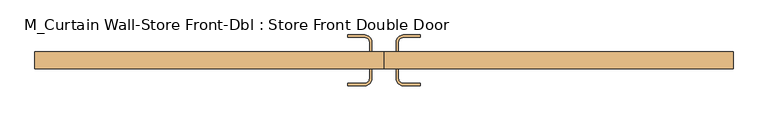
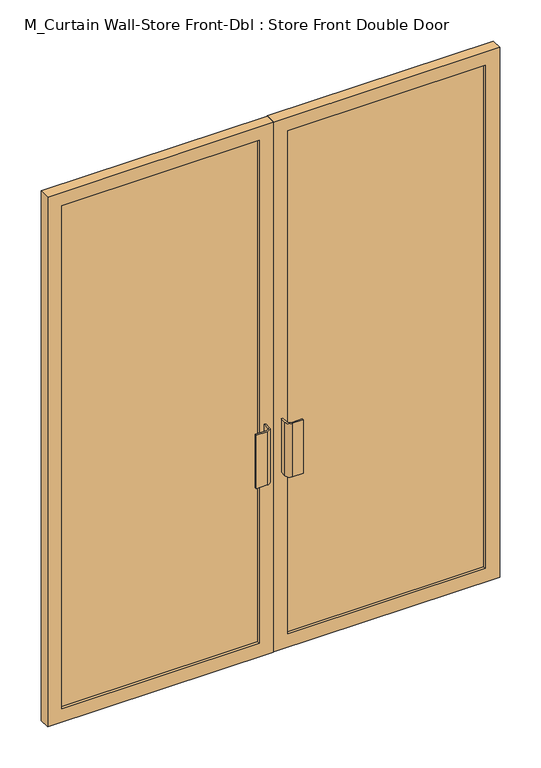
"""IFC4 building model written with IfcOpenShell, lengths in millimetres: door geometry, M_Curtain Wall-Store Front-Dbl : Store Front Double Door."""

import ifcopenshell
import ifcopenshell.guid

model = None  # the IFC model being written
_history = None  # IfcOwnerHistory: only IFC2X3 demands one
_inside = {}  # id of a spatial element -> (the spatial element, [elements in it])
_under = {}  # id of a project, library or spatial element -> (it, [spatial elements below it])
_declared = {}  # id of a project -> (the project, [libraries it declares])
_typed = {}  # id of a type object -> (the type object, [elements of that type])
_made_of = {}  # id of a material, layer set ... -> (it, [elements and type objects made of it])


def new_model(schema):
    """Start an empty IFC model of exactly this schema.

    Asked for "IFC4X3", IfcOpenShell would pick the latest addendum, in which some entities
    have other attributes; the version numbers below select the first issue.
    IFC2X3 requires an IfcOwnerHistory on every rooted entity: one is made here for all.
    """
    global model, _history
    if schema == "IFC4X3":
        model = ifcopenshell.file(schema_version=(4, 3, 0, 0))
    else:
        model = ifcopenshell.file(schema=schema)
    _inside.clear()
    _under.clear()
    _declared.clear()
    _typed.clear()
    _made_of.clear()
    _history = None
    if model.schema == "IFC2X3":
        org = make("IfcOrganization", Name="unknown")
        user = make(
            "IfcPersonAndOrganization",
            ThePerson=make("IfcPerson", FamilyName="unknown"),
            TheOrganization=org,
        )
        app = make(
            "IfcApplication",
            ApplicationDeveloper=org,
            Version="unknown",
            ApplicationFullName="unknown",
            ApplicationIdentifier="unknown",
        )
        _history = make(
            "IfcOwnerHistory",
            OwningUser=user,
            OwningApplication=app,
            ChangeAction="ADDED",
            CreationDate=0,
        )
    return model


def make(cls, **values):
    """One entity of the class cls with the attributes given. An attribute that is None is left unset."""
    return model.create_entity(
        cls, **{name: value for name, value in values.items() if value is not None}
    )


def rooted(cls, **values):
    """An entity with a GlobalId (a new one), such as an element, a storey or a relation."""
    return make(cls, GlobalId=ifcopenshell.guid.new(), OwnerHistory=_history, **values)


def si_unit(unit_type, name, prefix=None):
    """IfcSIUnit, for example si_unit("LENGTHUNIT", "METRE", prefix="MILLI")."""
    return make("IfcSIUnit", UnitType=unit_type, Prefix=prefix, Name=name)


def assignment(units):
    """IfcUnitAssignment: the units of a project."""
    return None if units is None else make("IfcUnitAssignment", Units=units)


def point(xyz):
    """IfcCartesianPoint."""
    return None if xyz is None else make("IfcCartesianPoint", Coordinates=xyz)


def direction(xyz):
    """IfcDirection."""
    return None if xyz is None else make("IfcDirection", DirectionRatios=xyz)


def frame(location, z_axis=None, x_axis=None):
    """IfcAxis2Placement3D, a coordinate frame: its origin and axes. An axis left out is left unset."""
    return make(
        "IfcAxis2Placement3D",
        Location=point(location),
        Axis=direction(z_axis),
        RefDirection=direction(x_axis),
    )


def frame_2d(location, x_axis=None):
    """IfcAxis2Placement2D, a coordinate frame in the plane: its origin and x axis."""
    return make(
        "IfcAxis2Placement2D", Location=point(location), RefDirection=direction(x_axis)
    )


def origin():
    """The frame at (0, 0, 0) with its axes left unset."""
    return frame((0.0, 0.0, 0.0))


def place(relative_to, where):
    """IfcLocalPlacement: puts the frame where relative to a parent placement (None: the world)."""
    return make(
        "IfcLocalPlacement", PlacementRelTo=relative_to, RelativePlacement=where
    )


def context(
    kind, dimensions, precision=None, world=None, true_north=None, identifier=None
):
    """IfcGeometricRepresentationContext, for example the 3D "Model" context."""
    return make(
        "IfcGeometricRepresentationContext",
        ContextIdentifier=identifier,
        ContextType=kind,
        CoordinateSpaceDimension=dimensions,
        Precision=precision,
        WorldCoordinateSystem=world,
        TrueNorth=true_north,
    )


def project(units=None, contexts=None):
    """IfcProject with its units and contexts."""
    return rooted(
        "IfcProject",
        Name="project",
        RepresentationContexts=contexts,
        UnitsInContext=assignment(units),
    )


def spatial(cls, under=None, at=None, **own):
    """A site, building, storey or space (cls), placed at a placement, below another one or the project."""
    s = rooted(cls, ObjectPlacement=at, **own)
    if under is not None:
        _under.setdefault(under.id(), (under, []))[1].append(s)
    return s


def polyline(points):
    """IfcPolyline through the points."""
    return make("IfcPolyline", Points=[point(p) for p in points])


def circle_curve(where, radius):
    """IfcCircle in the frame where."""
    return make("IfcCircle", Position=where, Radius=radius)


def trimmed(basis, trim1, trim2, sense, master):
    """IfcTrimmedCurve: the piece of a basis curve between two trims."""
    return make(
        "IfcTrimmedCurve",
        BasisCurve=basis,
        Trim1=trim1,
        Trim2=trim2,
        SenseAgreement=sense,
        MasterRepresentation=master,
    )


def segment(curve, same_sense, transition):
    """IfcCompositeCurveSegment."""
    return make(
        "IfcCompositeCurveSegment",
        Transition=transition,
        SameSense=same_sense,
        ParentCurve=curve,
    )


def composite_curve(segments, self_intersect=None):
    """IfcCompositeCurve: segments joined end to end."""
    return make("IfcCompositeCurve", Segments=segments, SelfIntersect=self_intersect)


def outline(outer, holes=None, kind="AREA"):
    """IfcArbitraryClosedProfileDef: a profile drawn as a closed curve; with holes, ...WithVoids."""
    if holes is None:
        return make("IfcArbitraryClosedProfileDef", ProfileType=kind, OuterCurve=outer)
    return make(
        "IfcArbitraryProfileDefWithVoids",
        ProfileType=kind,
        OuterCurve=outer,
        InnerCurves=holes,
    )


def extrude(swept, where, along, depth):
    """IfcExtrudedAreaSolid: the profile swept, set in the frame where, extruded along a direction by depth."""
    return make(
        "IfcExtrudedAreaSolid",
        SweptArea=swept,
        Position=where,
        ExtrudedDirection=direction(along),
        Depth=depth,
    )


def shape(context_of_items, identifier, shape_type, items):
    """IfcShapeRepresentation: the items that make up one representation, for example the "Body"."""
    return make(
        "IfcShapeRepresentation",
        ContextOfItems=context_of_items,
        RepresentationIdentifier=identifier,
        RepresentationType=shape_type,
        Items=items,
    )


def source(mapping_origin, context_of_items, identifier, shape_type, items):
    """IfcRepresentationMap: a shape defined once, which mapped items show again and again."""
    return make(
        "IfcRepresentationMap",
        MappingOrigin=mapping_origin,
        MappedRepresentation=shape(context_of_items, identifier, shape_type, items),
    )


def transform(
    local_origin,
    x_axis=None,
    y_axis=None,
    z_axis=None,
    scale=None,
    scale2=None,
    scale3=None,
    uniform=True,
):
    """IfcCartesianTransformationOperator3D, or its non-uniform kind. x_axis, y_axis, z_axis: its Axis1, 2, 3."""
    if uniform:
        return make(
            "IfcCartesianTransformationOperator3D",
            Axis1=direction(x_axis),
            Axis2=direction(y_axis),
            LocalOrigin=point(local_origin),
            Scale=scale,
            Axis3=direction(z_axis),
        )
    return make(
        "IfcCartesianTransformationOperator3DnonUniform",
        Axis1=direction(x_axis),
        Axis2=direction(y_axis),
        LocalOrigin=point(local_origin),
        Scale=scale,
        Axis3=direction(z_axis),
        Scale2=scale2,
        Scale3=scale3,
    )


def mapped(mapping_source, mapping_target):
    """IfcMappedItem: shows the shape of a source again, moved by a transform."""
    return make(
        "IfcMappedItem", MappingSource=mapping_source, MappingTarget=mapping_target
    )


def made_of(thing, what):
    """Note that an element or type object is made of a material, layer set ...; save() writes the relation."""
    if what is not None:
        _made_of.setdefault(what.id(), (what, []))[1].append(thing)
    return thing


def element(
    cls,
    number,
    at=None,
    inside=None,
    cuts=None,
    type_object=None,
    material=None,
    context=None,
    identifier="Body",
    shape_type=None,
    held_by="IfcProductDefinitionShape",
    body=None,
    shapes=None,
    **own,
):
    """One element of the class cls, such as IfcWall. Its Tag is "e" and its number.

    at: its placement. inside: the storey or other place that contains it. cuts: it is an
    opening in that element (IfcRelVoidsElement). A single representation is given by context,
    identifier, shape_type and body (its items); several are given by shapes. held_by: the class
    of the entity that holds the representations. save() writes the other relations.
    """
    e = rooted(cls, Tag="e%d" % number, ObjectPlacement=at, **own)
    if body is not None:
        shapes = [shape(context, identifier, shape_type, body)]
    if shapes is not None:
        e.Representation = make(held_by, Representations=shapes)
    if inside is not None:
        _inside.setdefault(inside.id(), (inside, []))[1].append(e)
    if cuts is not None:
        rooted(
            "IfcRelVoidsElement", RelatingBuildingElement=cuts, RelatedOpeningElement=e
        )
    if type_object is not None:
        _typed.setdefault(type_object.id(), (type_object, []))[1].append(e)
    return made_of(e, material)


def aggregate(whole, parts):
    """IfcRelAggregates: a whole, such as a stair, and the parts it consists of."""
    return rooted("IfcRelAggregates", RelatingObject=whole, RelatedObjects=parts)


def save(model, path):
    """Write the relations noted so far, then the file.

    IfcRelAggregates (storeys below a building ...), IfcRelContainedInSpatialStructure (elements
    in a storey), IfcRelDefinesByType, IfcRelAssociatesMaterial and IfcRelDeclares: one each for
    every whole, place, type object, material and project.
    """
    for whole, parts in _under.values():
        aggregate(whole, parts)
    for where, things in _inside.values():
        rooted(
            "IfcRelContainedInSpatialStructure",
            RelatedElements=things,
            RelatingStructure=where,
        )
    for kind, things in _typed.values():
        rooted("IfcRelDefinesByType", RelatedObjects=things, RelatingType=kind)
    for what, things in _made_of.values():
        rooted("IfcRelAssociatesMaterial", RelatedObjects=things, RelatingMaterial=what)
    for by, libraries in _declared.values():
        rooted("IfcRelDeclares", RelatingContext=by, RelatedDefinitions=libraries)
    model.write(path)


def m_curtain_wall_store_front_dbl_store_front_double_door_46208f06(model_context):
    return source(origin(), model_context, "Body", "SweptSolid", [
        extrude(outline(composite_curve([segment(trimmed(circle_curve(frame_2d((-50.8, -14.85)), 19.05), [point((-31.75, -14.85))], [point((-50.8, -33.9))], False, "CARTESIAN"), True, "CONTINUOUS"), segment(polyline([(-50.8, -33.9), (-95.25, -33.9), (-95.25, -27.55), (-50.8, -27.55)]), True, "CONTINUOUS"), segment(trimmed(circle_curve(frame_2d((-50.8, -14.85)), 12.7), [point((-50.8, -27.55))], [point((-38.1, -14.85))], True, "CARTESIAN"), True, "CONTINUOUS"), segment(polyline([(-38.1, -14.85), (-38.1, 10.55), (-31.75, 10.55), (-31.75, -14.85)]), True, "CONTINUOUS")], self_intersect=False)), frame((0.0, 0.0, 762.0), z_axis=(0.0, 0.0, 1.0), x_axis=(1.0, 0.0, 0.0)), (0.0, 0.0, 1.0), 228.6),
        extrude(outline(composite_curve([segment(polyline([(31.75, -14.85), (31.75, 10.55), (38.1, 10.55), (38.1, -14.85)]), True, "CONTINUOUS"), segment(trimmed(circle_curve(frame_2d((50.8, -14.85)), 12.7), [point((38.1, -14.85))], [point((50.8, -27.55))], True, "CARTESIAN"), True, "CONTINUOUS"), segment(polyline([(50.8, -27.55), (95.25, -27.55), (95.25, -33.9), (50.8, -33.9)]), True, "CONTINUOUS"), segment(trimmed(circle_curve(frame_2d((50.8, -14.85)), 19.05), [point((50.8, -33.9))], [point((31.75, -14.85))], False, "CARTESIAN"), True, "CONTINUOUS")], self_intersect=False)), frame((0.0, 0.0, 762.0), z_axis=(0.0, 0.0, 1.0), x_axis=(1.0, 0.0, 0.0)), (0.0, 0.0, 1.0), 228.6),
        extrude(outline(composite_curve([segment(polyline([(-31.75, 80.4), (-31.75, 55.0), (-38.1, 55.0), (-38.1, 80.4)]), True, "CONTINUOUS"), segment(trimmed(circle_curve(frame_2d((-50.8, 80.4)), 12.7), [point((-38.1, 80.4))], [point((-50.8, 93.1))], True, "CARTESIAN"), True, "CONTINUOUS"), segment(polyline([(-50.8, 93.1), (-95.25, 93.1), (-95.25, 99.45), (-50.8, 99.45)]), True, "CONTINUOUS"), segment(trimmed(circle_curve(frame_2d((-50.8, 80.4)), 19.05), [point((-50.8, 99.45))], [point((-31.75, 80.4))], False, "CARTESIAN"), True, "CONTINUOUS")], self_intersect=False)), frame((0.0, 0.0, 762.0), z_axis=(0.0, 0.0, 1.0), x_axis=(1.0, 0.0, 0.0)), (0.0, 0.0, 1.0), 228.6),
        extrude(outline(composite_curve([segment(trimmed(circle_curve(frame_2d((50.8, 80.4)), 19.05), [point((31.75, 80.4))], [point((50.8, 99.45))], False, "CARTESIAN"), True, "CONTINUOUS"), segment(polyline([(50.8, 99.45), (95.25, 99.45), (95.25, 93.1), (50.8, 93.1)]), True, "CONTINUOUS"), segment(trimmed(circle_curve(frame_2d((50.8, 80.4)), 12.7), [point((50.8, 93.1))], [point((38.1, 80.4))], True, "CARTESIAN"), True, "CONTINUOUS"), segment(polyline([(38.1, 80.4), (38.1, 55.0), (31.75, 55.0), (31.75, 80.4)]), True, "CONTINUOUS")], self_intersect=False)), frame((0.0, 0.0, 762.0), z_axis=(0.0, 0.0, 1.0), x_axis=(1.0, 0.0, 0.0)), (0.0, 0.0, 1.0), 228.6),
        extrude(outline(polyline([(860.9333333, 23.25), (57.94375, 23.25), (57.94375, 42.3), (860.9333333, 42.3), (860.9333333, 23.25)])), frame((0.0, 0.0, 57.15), z_axis=(0.0, 0.0, 1.0), x_axis=(1.0, 0.0, 0.0)), (0.0, 0.0, 1.0), 2160.7),
        extrude(outline(polyline([(-57.94375, 23.25), (-860.9333333, 23.25), (-860.9333333, 42.3), (-57.94375, 42.3), (-57.94375, 23.25)])), frame((0.0, 0.0, 57.15), z_axis=(0.0, 0.0, 1.0), x_axis=(1.0, 0.0, 0.0)), (0.0, 0.0, 1.0), 2160.7),
        extrude(outline(polyline([(2275.0, 0.79375), (0.0, 0.79375), (0.0, 918.0833333), (2275.0, 918.0833333), (2275.0, 0.79375)]), holes=[polyline([(2217.85, 57.94375), (2217.85, 860.9333333), (57.15, 860.9333333), (57.15, 57.94375), (2217.85, 57.94375)])]), frame((0.0, 10.55, 0.0), z_axis=(0.0, 1.0, 0.0), x_axis=(0.0, 0.0, 1.0)), (0.0, 0.0, 1.0), 44.45),
        extrude(outline(polyline([(2275.0, -0.79375), (2275.0, -918.0833333), (0.0, -918.0833333), (0.0, -0.79375), (2275.0, -0.79375)]), holes=[polyline([(2217.85, -860.9333333), (2217.85, -57.94375), (57.15, -57.94375), (57.15, -860.9333333), (2217.85, -860.9333333)])]), frame((0.0, 10.55, 0.0), z_axis=(0.0, 1.0, 0.0), x_axis=(0.0, 0.0, 1.0)), (0.0, 0.0, 1.0), 44.45),
    ])


if __name__ == "__main__":
    model = new_model("IFC4")
    model_context = context("Model", 3, world=origin())
    ifc_project = project(units=[si_unit("LENGTHUNIT", "METRE", prefix="MILLI")], contexts=[model_context])
    site = spatial("IfcSite", under=ifc_project)
    building = spatial("IfcBuilding", under=site)
    placement = place(None, origin())
    m_curtain_wall_store_front_dbl_store_front_double_door_shape = m_curtain_wall_store_front_dbl_store_front_double_door_46208f06(model_context)
    element("IfcDoor", 1, ObjectType="M_Curtain Wall-Store Front-Dbl : Store Front Double Door", at=placement, inside=building, context=model_context, shape_type="MappedRepresentation", body=[
        mapped(m_curtain_wall_store_front_dbl_store_front_double_door_shape, transform((0.0, 0.0, 0.0), x_axis=(1.0, 0.0, 0.0), y_axis=(0.0, 1.0, 0.0), z_axis=(0.0, 0.0, 1.0))),
    ])
    save(model, "model.ifc")

# Revit data of these elements
# Type "M_Curtain Wall-Store Front-Dbl : Store Front Double Door"
#   Type Mark = "35"
#   Offset = 0.055 m
#   Function = 1
#   Define Thermal Properties by = 1
#   Material = Metal - Aluminum
#   Glazing Material = Window - Glass
#   Assembly Code = ""
# Element 1 (IfcDoor, "M_Curtain Wall-Store Front-Dbl : Store Front Double Door")
#   Materials on its faces: "Metal - Aluminum", "Window - Glass"
# Materials
#   "Metal - Aluminum": class "Unassigned", colour RGB 247 247 247, transparency 0, Comments = "Rendering appearance not upgraded "
#   "Window - Glass": class "Glas", colour RGB 128 128 255, transparency 0.75
